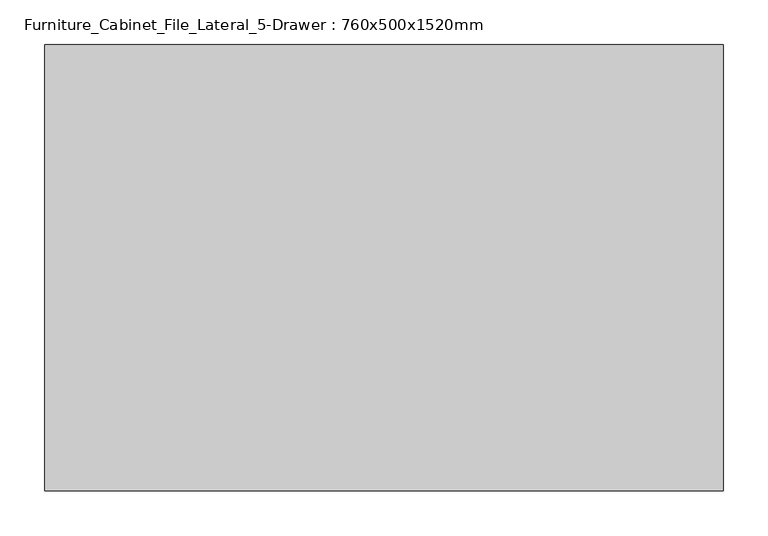
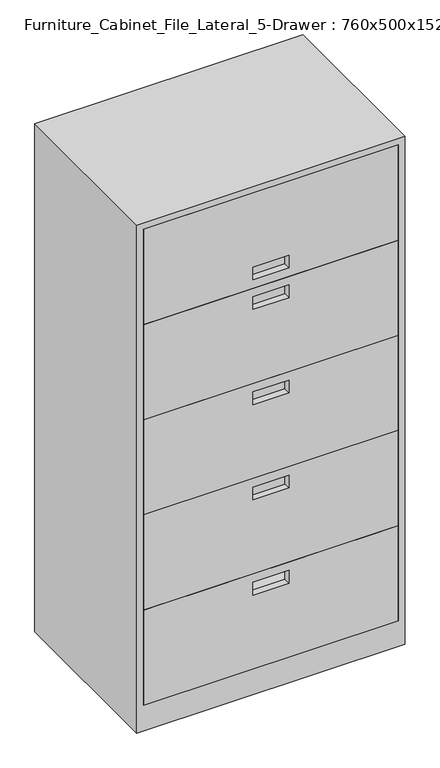
"""IFC4 building model written with IfcOpenShell, lengths in millimetres: furniture geometry, Furniture_Cabinet_File_Lateral_5-Drawer : 760x500x1520mm."""

from ifc_helpers import new_model, si_unit, frame, origin, place, context, project, spatial, polyline, outline, extrude, faceted_brep, source, transform, mapped, element, save


def furniture_cabinet_file_lateral_5_drawer_760x500x1520mm_9a48b8a7(model_context):
    return source(origin(), model_context, "Body", "SolidModel", [
        extrude(outline(polyline([(76.2, -540.9725139), (76.2, 180.9274861), (361.15, 180.9274861), (361.15, -540.9725139), (76.2, -540.9725139)]), holes=[polyline([(335.75, -230.8225139), (335.75, -129.2225139), (297.65, -129.2225139), (297.65, -230.8225139), (335.75, -230.8225139)])]), frame((0.0, -1184.3183761, 0.0), z_axis=(0.0, 1.0, 0.0), x_axis=(0.0, 0.0, 1.0)), (0.0, 0.0, 1.0), 19.05),
        extrude(outline(polyline([(361.15, -540.9725139), (361.15, 180.9274861), (646.1, 180.9274861), (646.1, -540.9725139), (361.15, -540.9725139)]), holes=[polyline([(620.7, -230.8225139), (620.7, -129.2225139), (582.6, -129.2225139), (582.6, -230.8225139), (620.7, -230.8225139)])]), frame((0.0, -1184.3183761, 0.0), z_axis=(0.0, 1.0, 0.0), x_axis=(0.0, 0.0, 1.0)), (0.0, 0.0, 1.0), 19.05),
        extrude(outline(polyline([(1500.95, -540.9725139), (1216.0, -540.9725139), (1216.0, 180.9274861), (1500.95, 180.9274861), (1500.95, -540.9725139)]), holes=[polyline([(1279.5, -129.2225139), (1241.4, -129.2225139), (1241.4, -230.8225139), (1279.5, -230.8225139), (1279.5, -129.2225139)])]), frame((0.0, -1184.3183761, 0.0), z_axis=(0.0, 1.0, 0.0), x_axis=(0.0, 0.0, 1.0)), (0.0, 0.0, 1.0), 19.05),
        extrude(outline(polyline([(1216.0, -540.9725139), (931.05, -540.9725139), (931.05, 180.9274861), (1216.0, 180.9274861), (1216.0, -540.9725139)]), holes=[polyline([(1190.6, -230.8225139), (1190.6, -129.2225139), (1152.5, -129.2225139), (1152.5, -230.8225139), (1190.6, -230.8225139)])]), frame((0.0, -1184.3183761, 0.0), z_axis=(0.0, 1.0, 0.0), x_axis=(0.0, 0.0, 1.0)), (0.0, 0.0, 1.0), 19.05),
        extrude(outline(polyline([(931.05, -540.9725139), (646.1, -540.9725139), (646.1, 180.9274861), (931.05, 180.9274861), (931.05, -540.9725139)]), holes=[polyline([(905.65, -230.8225139), (905.65, -129.2225139), (867.55, -129.2225139), (867.55, -230.8225139), (905.65, -230.8225139)])]), frame((0.0, -1184.3183761, 0.0), z_axis=(0.0, 1.0, 0.0), x_axis=(0.0, 0.0, 1.0)), (0.0, 0.0, 1.0), 19.05),
        faceted_brep([(199.9774861, -684.3183761, 1520.0), (-560.0225139, -684.3183761, 1520.0), (-560.0225139, -1184.3183761, 1520.0), (199.9774861, -1184.3183761, 1520.0), (199.9774861, -684.3183761, 0.0), (199.9774861, -1184.3183761, 0.0), (-560.0225139, -1184.3183761, 0.0), (-560.0225139, -684.3183761, 0.0), (180.9274861, -1184.3183761, 76.2), (-540.9725139, -1184.3183761, 76.2), (-540.9725139, -1184.3183761, 1500.95), (180.9274861, -1184.3183761, 1500.95), (-540.9725139, -703.3683761, 76.2), (180.9274861, -703.3683761, 76.2), (180.9274861, -703.3683761, 1500.95), (-540.9725139, -703.3683761, 1500.95)], [[[0, 1, 2, 3]], [[4, 5, 6, 7]], [[1, 0, 4, 7]], [[2, 1, 7, 6]], [[3, 2, 6, 5], [8, 9, 10, 11]], [[0, 3, 5, 4]], [[12, 13, 14, 15]], [[13, 12, 9, 8]], [[14, 13, 8, 11]], [[15, 14, 11, 10]], [[12, 15, 10, 9]]]),
    ])


if __name__ == "__main__":
    model = new_model("IFC4")
    model_context = context("Model", 3, world=origin())
    ifc_project = project(units=[si_unit("LENGTHUNIT", "METRE", prefix="MILLI")], contexts=[model_context])
    site = spatial("IfcSite", under=ifc_project)
    building = spatial("IfcBuilding", under=site)
    placement = place(None, origin())
    furniture_cabinet_file_lateral_5_drawer_760x500x1520mm_shape = furniture_cabinet_file_lateral_5_drawer_760x500x1520mm_9a48b8a7(model_context)
    element("IfcFurniture", 1, ObjectType="Furniture_Cabinet_File_Lateral_5-Drawer : 760x500x1520mm", at=placement, inside=building, context=model_context, shape_type="MappedRepresentation", body=[
        mapped(furniture_cabinet_file_lateral_5_drawer_760x500x1520mm_shape, transform((0.0, 0.0, 0.0), x_axis=(1.0, 0.0, 0.0), y_axis=(0.0, 1.0, 0.0), z_axis=(0.0, 0.0, 1.0))),
    ])
    save(model, "model.ifc")

# Revit data of these elements
# Type "Furniture_Cabinet_File_Lateral_5-Drawer : 760x500x1520mm"
#   Keynote = "N"
#   Assembly Code = "E2020200"
#   Depth = 500 mm
#   Height = 1520 mm
#   Width = 760 mm
#   Material = Metal - Steel
#   Default Elevation = 0
# Element 1 (IfcFurniture, "Furniture_Cabinet_File_Lateral_5-Drawer : 760x500x1520mm")
#   Materials on its faces: "Metal - Steel"
# Materials
#   "Metal - Steel": class "Metal", colour RGB 247 247 247, transparency 0
